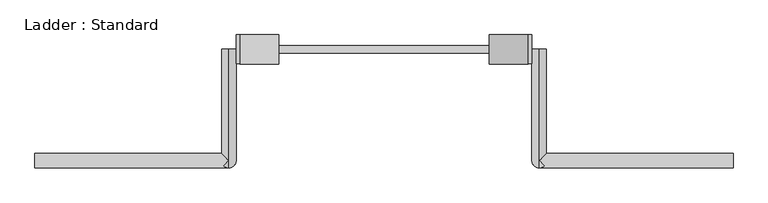
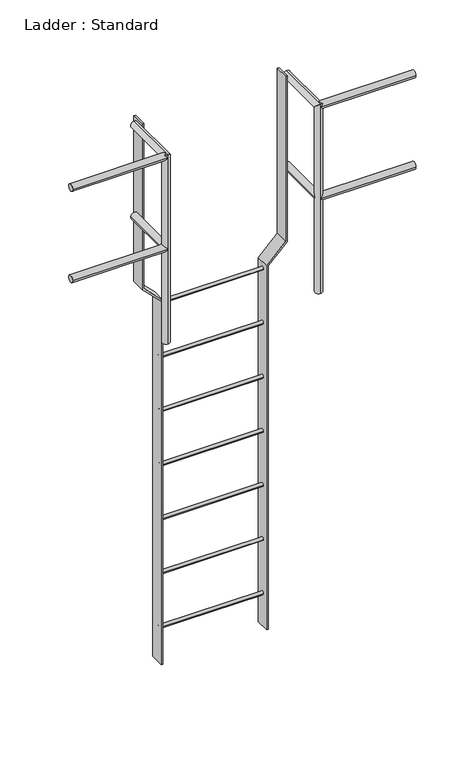
"""IFC4 building model written with IfcOpenShell, lengths in millimetres: proxy geometry, Ladder : Standard."""

import ifcopenshell
import ifcopenshell.guid

model = None  # the IFC model being written
_history = None  # IfcOwnerHistory: only IFC2X3 demands one
_inside = {}  # id of a spatial element -> (the spatial element, [elements in it])
_under = {}  # id of a project, library or spatial element -> (it, [spatial elements below it])
_declared = {}  # id of a project -> (the project, [libraries it declares])
_typed = {}  # id of a type object -> (the type object, [elements of that type])
_made_of = {}  # id of a material, layer set ... -> (it, [elements and type objects made of it])


def new_model(schema):
    """Start an empty IFC model of exactly this schema.

    Asked for "IFC4X3", IfcOpenShell would pick the latest addendum, in which some entities
    have other attributes; the version numbers below select the first issue.
    IFC2X3 requires an IfcOwnerHistory on every rooted entity: one is made here for all.
    """
    global model, _history
    if schema == "IFC4X3":
        model = ifcopenshell.file(schema_version=(4, 3, 0, 0))
    else:
        model = ifcopenshell.file(schema=schema)
    _inside.clear()
    _under.clear()
    _declared.clear()
    _typed.clear()
    _made_of.clear()
    _history = None
    if model.schema == "IFC2X3":
        org = make("IfcOrganization", Name="unknown")
        user = make(
            "IfcPersonAndOrganization",
            ThePerson=make("IfcPerson", FamilyName="unknown"),
            TheOrganization=org,
        )
        app = make(
            "IfcApplication",
            ApplicationDeveloper=org,
            Version="unknown",
            ApplicationFullName="unknown",
            ApplicationIdentifier="unknown",
        )
        _history = make(
            "IfcOwnerHistory",
            OwningUser=user,
            OwningApplication=app,
            ChangeAction="ADDED",
            CreationDate=0,
        )
    return model


def make(cls, **values):
    """One entity of the class cls with the attributes given. An attribute that is None is left unset."""
    return model.create_entity(
        cls, **{name: value for name, value in values.items() if value is not None}
    )


def rooted(cls, **values):
    """An entity with a GlobalId (a new one), such as an element, a storey or a relation."""
    return make(cls, GlobalId=ifcopenshell.guid.new(), OwnerHistory=_history, **values)


def si_unit(unit_type, name, prefix=None):
    """IfcSIUnit, for example si_unit("LENGTHUNIT", "METRE", prefix="MILLI")."""
    return make("IfcSIUnit", UnitType=unit_type, Prefix=prefix, Name=name)


def assignment(units):
    """IfcUnitAssignment: the units of a project."""
    return None if units is None else make("IfcUnitAssignment", Units=units)


def point(xyz):
    """IfcCartesianPoint."""
    return None if xyz is None else make("IfcCartesianPoint", Coordinates=xyz)


def direction(xyz):
    """IfcDirection."""
    return None if xyz is None else make("IfcDirection", DirectionRatios=xyz)


def frame(location, z_axis=None, x_axis=None):
    """IfcAxis2Placement3D, a coordinate frame: its origin and axes. An axis left out is left unset."""
    return make(
        "IfcAxis2Placement3D",
        Location=point(location),
        Axis=direction(z_axis),
        RefDirection=direction(x_axis),
    )


def frame_2d(location, x_axis=None):
    """IfcAxis2Placement2D, a coordinate frame in the plane: its origin and x axis."""
    return make(
        "IfcAxis2Placement2D", Location=point(location), RefDirection=direction(x_axis)
    )


def origin():
    """The frame at (0, 0, 0) with its axes left unset."""
    return frame((0.0, 0.0, 0.0))


def place(relative_to, where):
    """IfcLocalPlacement: puts the frame where relative to a parent placement (None: the world)."""
    return make(
        "IfcLocalPlacement", PlacementRelTo=relative_to, RelativePlacement=where
    )


def context(
    kind, dimensions, precision=None, world=None, true_north=None, identifier=None
):
    """IfcGeometricRepresentationContext, for example the 3D "Model" context."""
    return make(
        "IfcGeometricRepresentationContext",
        ContextIdentifier=identifier,
        ContextType=kind,
        CoordinateSpaceDimension=dimensions,
        Precision=precision,
        WorldCoordinateSystem=world,
        TrueNorth=true_north,
    )


def project(units=None, contexts=None):
    """IfcProject with its units and contexts."""
    return rooted(
        "IfcProject",
        Name="project",
        RepresentationContexts=contexts,
        UnitsInContext=assignment(units),
    )


def spatial(cls, under=None, at=None, **own):
    """A site, building, storey or space (cls), placed at a placement, below another one or the project."""
    s = rooted(cls, ObjectPlacement=at, **own)
    if under is not None:
        _under.setdefault(under.id(), (under, []))[1].append(s)
    return s


def polyline(points):
    """IfcPolyline through the points."""
    return make("IfcPolyline", Points=[point(p) for p in points])


def circle_curve(where, radius):
    """IfcCircle in the frame where."""
    return make("IfcCircle", Position=where, Radius=radius)


def ellipse_curve(where, semi_axis1, semi_axis2):
    """IfcEllipse in the frame where."""
    return make(
        "IfcEllipse", Position=where, SemiAxis1=semi_axis1, SemiAxis2=semi_axis2
    )


def trimmed(basis, trim1, trim2, sense, master):
    """IfcTrimmedCurve: the piece of a basis curve between two trims."""
    return make(
        "IfcTrimmedCurve",
        BasisCurve=basis,
        Trim1=trim1,
        Trim2=trim2,
        SenseAgreement=sense,
        MasterRepresentation=master,
    )


def segment(curve, same_sense, transition):
    """IfcCompositeCurveSegment."""
    return make(
        "IfcCompositeCurveSegment",
        Transition=transition,
        SameSense=same_sense,
        ParentCurve=curve,
    )


def composite_curve(segments, self_intersect=None):
    """IfcCompositeCurve: segments joined end to end."""
    return make("IfcCompositeCurve", Segments=segments, SelfIntersect=self_intersect)


def outline(outer, holes=None, kind="AREA"):
    """IfcArbitraryClosedProfileDef: a profile drawn as a closed curve; with holes, ...WithVoids."""
    if holes is None:
        return make("IfcArbitraryClosedProfileDef", ProfileType=kind, OuterCurve=outer)
    return make(
        "IfcArbitraryProfileDefWithVoids",
        ProfileType=kind,
        OuterCurve=outer,
        InnerCurves=holes,
    )


def extrude(swept, where, along, depth):
    """IfcExtrudedAreaSolid: the profile swept, set in the frame where, extruded along a direction by depth."""
    return make(
        "IfcExtrudedAreaSolid",
        SweptArea=swept,
        Position=where,
        ExtrudedDirection=direction(along),
        Depth=depth,
    )


def shape(context_of_items, identifier, shape_type, items):
    """IfcShapeRepresentation: the items that make up one representation, for example the "Body"."""
    return make(
        "IfcShapeRepresentation",
        ContextOfItems=context_of_items,
        RepresentationIdentifier=identifier,
        RepresentationType=shape_type,
        Items=items,
    )


def source(mapping_origin, context_of_items, identifier, shape_type, items):
    """IfcRepresentationMap: a shape defined once, which mapped items show again and again."""
    return make(
        "IfcRepresentationMap",
        MappingOrigin=mapping_origin,
        MappedRepresentation=shape(context_of_items, identifier, shape_type, items),
    )


def transform(
    local_origin,
    x_axis=None,
    y_axis=None,
    z_axis=None,
    scale=None,
    scale2=None,
    scale3=None,
    uniform=True,
):
    """IfcCartesianTransformationOperator3D, or its non-uniform kind. x_axis, y_axis, z_axis: its Axis1, 2, 3."""
    if uniform:
        return make(
            "IfcCartesianTransformationOperator3D",
            Axis1=direction(x_axis),
            Axis2=direction(y_axis),
            LocalOrigin=point(local_origin),
            Scale=scale,
            Axis3=direction(z_axis),
        )
    return make(
        "IfcCartesianTransformationOperator3DnonUniform",
        Axis1=direction(x_axis),
        Axis2=direction(y_axis),
        LocalOrigin=point(local_origin),
        Scale=scale,
        Axis3=direction(z_axis),
        Scale2=scale2,
        Scale3=scale3,
    )


def mapped(mapping_source, mapping_target):
    """IfcMappedItem: shows the shape of a source again, moved by a transform."""
    return make(
        "IfcMappedItem", MappingSource=mapping_source, MappingTarget=mapping_target
    )


def made_of(thing, what):
    """Note that an element or type object is made of a material, layer set ...; save() writes the relation."""
    if what is not None:
        _made_of.setdefault(what.id(), (what, []))[1].append(thing)
    return thing


def element(
    cls,
    number,
    at=None,
    inside=None,
    cuts=None,
    type_object=None,
    material=None,
    context=None,
    identifier="Body",
    shape_type=None,
    held_by="IfcProductDefinitionShape",
    body=None,
    shapes=None,
    **own,
):
    """One element of the class cls, such as IfcWall. Its Tag is "e" and its number.

    at: its placement. inside: the storey or other place that contains it. cuts: it is an
    opening in that element (IfcRelVoidsElement). A single representation is given by context,
    identifier, shape_type and body (its items); several are given by shapes. held_by: the class
    of the entity that holds the representations. save() writes the other relations.
    """
    e = rooted(cls, Tag="e%d" % number, ObjectPlacement=at, **own)
    if body is not None:
        shapes = [shape(context, identifier, shape_type, body)]
    if shapes is not None:
        e.Representation = make(held_by, Representations=shapes)
    if inside is not None:
        _inside.setdefault(inside.id(), (inside, []))[1].append(e)
    if cuts is not None:
        rooted(
            "IfcRelVoidsElement", RelatingBuildingElement=cuts, RelatedOpeningElement=e
        )
    if type_object is not None:
        _typed.setdefault(type_object.id(), (type_object, []))[1].append(e)
    return made_of(e, material)


def aggregate(whole, parts):
    """IfcRelAggregates: a whole, such as a stair, and the parts it consists of."""
    return rooted("IfcRelAggregates", RelatingObject=whole, RelatedObjects=parts)


def save(model, path):
    """Write the relations noted so far, then the file.

    IfcRelAggregates (storeys below a building ...), IfcRelContainedInSpatialStructure (elements
    in a storey), IfcRelDefinesByType, IfcRelAssociatesMaterial and IfcRelDeclares: one each for
    every whole, place, type object, material and project.
    """
    for whole, parts in _under.values():
        aggregate(whole, parts)
    for where, things in _inside.values():
        rooted(
            "IfcRelContainedInSpatialStructure",
            RelatedElements=things,
            RelatingStructure=where,
        )
    for kind, things in _typed.values():
        rooted("IfcRelDefinesByType", RelatedObjects=things, RelatingType=kind)
    for what, things in _made_of.values():
        rooted("IfcRelAssociatesMaterial", RelatedObjects=things, RelatingMaterial=what)
    for by, libraries in _declared.values():
        rooted("IfcRelDeclares", RelatingContext=by, RelatedDefinitions=libraries)
    model.write(path)


def plane_surface(at):
    """IfcPlane: the flat surface through the origin of the frame at, square to its z axis."""
    return make("IfcPlane", Position=at)


def cylinder_surface(at, radius):
    """IfcCylindricalSurface: all points at the distance radius from the z axis of the frame at."""
    return make("IfcCylindricalSurface", Position=at, Radius=radius)


def advanced_brep(points, edges, surfaces, faces):
    """IfcAdvancedBrep: a solid bounded by faces that lie on surfaces and meet in shared edges.

    An edge is (start, end): straight between two places in points (the first is 0);
    or (start, end, curve); or (start, end, curve, False) where it runs against its curve.
    A face is (place in surfaces, loops), or (place, loops, False) where it looks against
    its surface's normal. A loop lists edges by number (the first is 1), with a minus sign
    where the edge is run from its end to its start. The first loop is the outer one.
    """
    corners = [point(p) for p in points]
    vertices = [make("IfcVertexPoint", VertexGeometry=c) for c in corners]
    made = []
    for start, end, *more in edges:
        made.append(
            make(
                "IfcEdgeCurve",
                EdgeStart=vertices[start],
                EdgeEnd=vertices[end],
                EdgeGeometry=more[0] if more else make("IfcPolyline", Points=[corners[start], corners[end]]),
                SameSense=more[1] if len(more) > 1 else True,
            )
        )
    hull = []
    for where, loops, *sense in faces:
        bounds = []
        for j, loop in enumerate(loops):
            ring = [make("IfcOrientedEdge", EdgeElement=made[abs(k) - 1], Orientation=k > 0) for k in loop]
            bounds.append(
                make(
                    "IfcFaceOuterBound" if j == 0 else "IfcFaceBound",
                    Bound=make("IfcEdgeLoop", EdgeList=ring),
                    Orientation=True,
                )
            )
        hull.append(make("IfcAdvancedFace", Bounds=bounds, FaceSurface=surfaces[where], SameSense=sense[0] if sense else True))
    return make("IfcAdvancedBrep", Outer=make("IfcClosedShell", CfsFaces=hull))


def ladder_standard_c970834c(model_context):
    return source(origin(), model_context, "Body", "SolidModel", [
        extrude(outline(composite_curve([segment(trimmed(circle_curve(frame_2d((292.1, -1828.8)), 9.525), [point((282.575, -1828.8))], [point((301.625, -1828.8))], False, "CARTESIAN"), True, "CONTINUOUS"), segment(trimmed(circle_curve(frame_2d((292.1, -1828.8)), 9.525), [point((301.625, -1828.8))], [point((282.575, -1828.8))], False, "CARTESIAN"), True, "CONTINUOUS")], self_intersect=False)), frame((-276.3329351, 0.0, 0.0), z_axis=(1.0, 0.0, 0.0), x_axis=(0.0, 1.0, 0.0)), (0.0, 0.0, 1.0), 552.6658703),
        extrude(outline(composite_curve([segment(trimmed(circle_curve(frame_2d((292.1, -1524.0)), 9.525), [point((282.575, -1524.0))], [point((301.625, -1524.0))], False, "CARTESIAN"), True, "CONTINUOUS"), segment(trimmed(circle_curve(frame_2d((292.1, -1524.0)), 9.525), [point((301.625, -1524.0))], [point((282.575, -1524.0))], False, "CARTESIAN"), True, "CONTINUOUS")], self_intersect=False)), frame((-276.3329351, 0.0, 0.0), z_axis=(1.0, 0.0, 0.0), x_axis=(0.0, 1.0, 0.0)), (0.0, 0.0, 1.0), 552.6658703),
        extrude(outline(composite_curve([segment(trimmed(circle_curve(frame_2d((292.1, -1219.2)), 9.525), [point((282.575, -1219.2))], [point((301.625, -1219.2))], False, "CARTESIAN"), True, "CONTINUOUS"), segment(trimmed(circle_curve(frame_2d((292.1, -1219.2)), 9.525), [point((301.625, -1219.2))], [point((282.575, -1219.2))], False, "CARTESIAN"), True, "CONTINUOUS")], self_intersect=False)), frame((-276.3329351, 0.0, 0.0), z_axis=(1.0, 0.0, 0.0), x_axis=(0.0, 1.0, 0.0)), (0.0, 0.0, 1.0), 552.6658703),
        extrude(outline(composite_curve([segment(trimmed(circle_curve(frame_2d((292.1, -914.4)), 9.525), [point((282.575, -914.4))], [point((301.625, -914.4))], False, "CARTESIAN"), True, "CONTINUOUS"), segment(trimmed(circle_curve(frame_2d((292.1, -914.4)), 9.525), [point((301.625, -914.4))], [point((282.575, -914.4))], False, "CARTESIAN"), True, "CONTINUOUS")], self_intersect=False)), frame((-276.3329351, 0.0, 0.0), z_axis=(1.0, 0.0, 0.0), x_axis=(0.0, 1.0, 0.0)), (0.0, 0.0, 1.0), 552.6658703),
        extrude(outline(composite_curve([segment(trimmed(circle_curve(frame_2d((292.1, -609.6)), 9.525), [point((282.575, -609.6))], [point((301.625, -609.6))], False, "CARTESIAN"), True, "CONTINUOUS"), segment(trimmed(circle_curve(frame_2d((292.1, -609.6)), 9.525), [point((301.625, -609.6))], [point((282.575, -609.6))], False, "CARTESIAN"), True, "CONTINUOUS")], self_intersect=False)), frame((-276.3329351, 0.0, 0.0), z_axis=(1.0, 0.0, 0.0), x_axis=(0.0, 1.0, 0.0)), (0.0, 0.0, 1.0), 552.6658703),
        extrude(outline(composite_curve([segment(trimmed(circle_curve(frame_2d((292.1, -304.8)), 9.525), [point((282.575, -304.8))], [point((301.625, -304.8))], False, "CARTESIAN"), True, "CONTINUOUS"), segment(trimmed(circle_curve(frame_2d((292.1, -304.8)), 9.525), [point((301.625, -304.8))], [point((282.575, -304.8))], False, "CARTESIAN"), True, "CONTINUOUS")], self_intersect=False)), frame((-276.3329351, 0.0, 0.0), z_axis=(1.0, 0.0, 0.0), x_axis=(0.0, 1.0, 0.0)), (0.0, 0.0, 1.0), 552.6658703),
        extrude(outline(composite_curve([segment(trimmed(circle_curve(frame_2d((292.1, 0.0)), 9.525), [point((282.575, 0.0))], [point((301.625, 0.0))], False, "CARTESIAN"), True, "CONTINUOUS"), segment(trimmed(circle_curve(frame_2d((292.1, 0.0)), 9.525), [point((301.625, 0.0))], [point((282.575, 0.0))], False, "CARTESIAN"), True, "CONTINUOUS")], self_intersect=False)), frame((-276.3329351, 0.0, 0.0), z_axis=(1.0, 0.0, 0.0), x_axis=(0.0, 1.0, 0.0)), (0.0, 0.0, 1.0), 552.6658703),
        advanced_brep(
        [(387.4579351, 292.1, 533.4), (425.5579351, 292.1, 533.4), (425.5579351, 19.05, 533.4), (419.9783193, 13.4703842, 519.9296158), (406.5079351, 19.05, 514.35), (387.4579351, 0.0, 533.4), (406.5079351, 19.05, 552.45), (419.9783193, 13.4703842, 546.8703842), (914.5079351, -19.05, 533.4), (914.5079351, 19.05, 533.4), (406.5079351, -19.05, 533.4), (406.5079351, 19.05, 0.0), (406.5079351, -19.05, 0.0), (406.5079351, 19.05, 1028.7), (419.9783193, 13.4703842, 1034.2796158), (406.5079351, -19.05, 1047.75), (419.9783193, -13.4703842, 1061.2203842), (406.5079351, -19.05, 1066.8), (406.5079351, 292.1, 1028.7), (406.5079351, 292.1, 1066.8), (406.5079351, 0.0, 1066.8), (425.5579351, 19.05, 1047.75), (914.5079351, -19.05, 1047.75), (914.5079351, 19.05, 1047.75)],
        [
            (0, 1, circle_curve(frame((406.5079351, 292.1, 533.4), z_axis=(0.0, 1.0, 0.0), x_axis=(1.0, 0.0, 0.0)), 19.05)),
            (1, 0, circle_curve(frame((406.5079351, 292.1, 533.4), z_axis=(0.0, 1.0, 0.0), x_axis=(1.0, 0.0, 0.0)), 19.05)),
            (1, 2),
            (2, 3, ellipse_curve(frame((406.5079351, 0.0, 533.4), z_axis=(-0.7071067811865459, 0.7071067811865492, 0.0), x_axis=(-0.7071067811865492, -0.7071067811865457, 0.0)), 26.9407684, 19.05)),
            (3, 4, ellipse_curve(frame((406.5079351, 0.0, 533.4), z_axis=(0.0, 0.7071067811865475, 0.7071067811865475), x_axis=(0.0, -0.7071067811865476, 0.7071067811865474)), 26.9407684, 19.05)),
            (4, 5, ellipse_curve(frame((406.5079351, 0.0, 533.4), z_axis=(0.0, 0.7071067811865475, 0.7071067811865475), x_axis=(0.0, -0.7071067811865476, 0.7071067811865474)), 26.9407684, 19.05)),
            (5, 0),
            (5, 6, ellipse_curve(frame((406.5079351, 0.0, 533.4), z_axis=(0.0, 0.7071067811865475, -0.7071067811865475), x_axis=(0.0, -0.7071067811865476, -0.7071067811865474)), 26.9407684, 19.05)),
            (6, 7, ellipse_curve(frame((406.5079351, 0.0, 533.4), z_axis=(0.0, 0.7071067811865475, -0.7071067811865475), x_axis=(0.0, -0.7071067811865476, -0.7071067811865474)), 26.9407684, 19.05)),
            (7, 2, ellipse_curve(frame((406.5079351, 0.0, 533.4), z_axis=(-0.7071067811865459, 0.7071067811865492, 0.0), x_axis=(-0.7071067811865492, -0.7071067811865457, 0.0)), 26.9407684, 19.05)),
            (8, 9, circle_curve(frame((914.5079351, 0.0, 533.4), z_axis=(1.0, 0.0, 0.0), x_axis=(0.0, 1.0, 0.0)), 19.05)),
            (9, 8, circle_curve(frame((914.5079351, 0.0, 533.4), z_axis=(1.0, 0.0, 0.0), x_axis=(0.0, 1.0, 0.0)), 19.05)),
            (8, 10),
            (10, 3, ellipse_curve(frame((406.5079351, 0.0, 533.4), z_axis=(0.7071067811865475, 0.0, 0.7071067811865476), x_axis=(0.7071067811865476, 0.0, -0.7071067811865474)), 26.9407684, 19.05)),
            (2, 9),
            (7, 10, ellipse_curve(frame((406.5079351, 0.0, 533.4), z_axis=(0.7071067811865476, 0.0, -0.7071067811865475), x_axis=(0.7071067811865474, 0.0, 0.7071067811865476)), 26.9407684, 19.05)),
            (11, 12, circle_curve(frame((406.5079351, 0.0, 0.0), z_axis=(0.0, 0.0, -1.0), x_axis=(0.0, -1.0, 0.0)), 19.05)),
            (12, 11, circle_curve(frame((406.5079351, 0.0, 0.0), z_axis=(0.0, 0.0, -1.0), x_axis=(0.0, -1.0, 0.0)), 19.05)),
            (11, 4),
            (10, 12),
            (6, 13),
            (13, 14, ellipse_curve(frame((406.5079351, 0.0, 1047.75), z_axis=(0.0, -0.7071067811865475, -0.7071067811865475), x_axis=(0.0, 0.7071067811865474, -0.7071067811865476)), 26.9407684, 19.05)),
            (14, 15, ellipse_curve(frame((406.5079351, 0.0, 1047.75), z_axis=(-0.7071067811865475, 0.0, -0.7071067811865476), x_axis=(0.7071067811865476, 0.0, -0.7071067811865474)), 26.9407684, 19.05)),
            (15, 10),
            (16, 17, ellipse_curve(frame((406.5079351, 0.0, 1047.75), z_axis=(0.0, -0.7071067811865475, -0.7071067811865475), x_axis=(0.0, 0.7071067811865474, -0.7071067811865476)), 26.9407684, 19.05)),
            (17, 15),
            (15, 16, ellipse_curve(frame((406.5079351, 0.0, 1047.75), z_axis=(-0.7071067811865476, 0.0, 0.7071067811865475), x_axis=(-0.7071067811865474, 0.0, -0.7071067811865476)), 26.9407684, 19.05)),
            (17, 13, ellipse_curve(frame((406.5079351, 0.0, 1047.75), z_axis=(0.0, -0.7071067811865475, -0.7071067811865475), x_axis=(0.0, 0.7071067811865474, -0.7071067811865476)), 26.9407684, 19.05)),
            (18, 19, circle_curve(frame((406.5079351, 292.1, 1047.75), z_axis=(0.0, 1.0, 0.0), x_axis=(0.0, 0.0, 1.0)), 19.05)),
            (19, 18, circle_curve(frame((406.5079351, 292.1, 1047.75), z_axis=(0.0, 1.0, 0.0), x_axis=(0.0, 0.0, 1.0)), 19.05)),
            (16, 20, ellipse_curve(frame((406.5079351, 0.0, 1047.75), z_axis=(-0.7071067811865508, -0.7071067811865441, 0.0), x_axis=(0.7071067811865441, -0.7071067811865509, 0.0)), 26.9407684, 19.05)),
            (20, 17),
            (19, 20),
            (20, 21, ellipse_curve(frame((406.5079351, 0.0, 1047.75), z_axis=(-0.7071067811865441, 0.7071067811865508, 0.0), x_axis=(-0.7071067811865507, -0.7071067811865442, 0.0)), 26.9407684, 19.05)),
            (21, 14, ellipse_curve(frame((406.5079351, 0.0, 1047.75), z_axis=(-0.7071067811865441, 0.7071067811865508, 0.0), x_axis=(-0.7071067811865507, -0.7071067811865442, 0.0)), 26.9407684, 19.05)),
            (13, 18),
            (22, 23, circle_curve(frame((914.5079351, 0.0, 1047.75), z_axis=(1.0, 0.0, 0.0), x_axis=(0.0, 1.0, 0.0)), 19.05)),
            (23, 22, circle_curve(frame((914.5079351, 0.0, 1047.75), z_axis=(1.0, 0.0, 0.0), x_axis=(0.0, 1.0, 0.0)), 19.05)),
            (22, 15),
            (21, 23),
        ],
        [
            plane_surface(frame((425.5579351, 292.1, 533.4), z_axis=(0.0, 1.0, 0.0), x_axis=(0.0, 0.0, -1.0))),
            cylinder_surface(frame((406.5079351, 292.1, 533.4), z_axis=(0.0, -1.0, 0.0), x_axis=(1.0, 0.0, 0.0)), 19.05),
            plane_surface(frame((914.5079351, 19.05, 533.4), z_axis=(1.0, 0.0, 0.0), x_axis=(0.0, 0.0, 1.0))),
            cylinder_surface(frame((406.5079351, 0.0, 533.4), z_axis=(1.0, 0.0, 0.0), x_axis=(0.0, 1.0, 0.0)), 19.05),
            plane_surface(frame((0.0, 0.0, 0.0), z_axis=(0.0, 0.0, -1.0), x_axis=(1.0, 0.0, 0.0))),
            cylinder_surface(frame((406.5079351, 0.0, 0.0), z_axis=(0.0, 0.0, -1.0), x_axis=(0.0, -1.0, 0.0)), 19.05),
            plane_surface(frame((0.0, 292.1, 1047.75), z_axis=(0.0, 1.0, 0.0), x_axis=(1.0, 0.0, 0.0))),
            cylinder_surface(frame((406.5079351, 0.0, 1047.75), z_axis=(0.0, -1.0, 0.0), x_axis=(0.0, 0.0, 1.0)), 19.05),
            plane_surface(frame((914.5079351, 19.05, 1047.75), z_axis=(1.0, 0.0, 0.0), x_axis=(0.0, 0.0, 1.0))),
            cylinder_surface(frame((406.5079351, 0.0, 1047.75), z_axis=(1.0, 0.0, 0.0), x_axis=(0.0, 1.0, 0.0)), 19.05),
        ],
        [
            (0, [[1, 2]]),
            (1, [[-2, 3, 4, 5, 6, 7]]),
            (1, [[-1, -7, 8, 9, 10, -3]]),
            (2, [[11, 12]]),
            (3, [[-11, 13, 14, -4, 15]]),
            (3, [[-12, -15, -10, 16, -13]]),
            (4, [[17, 18]]),
            (5, [[-17, 19, -5, -14, 20]]),
            (5, [[21, 22, 23, 24, -16, -9]]),
            (5, [[25, 26, 27]]),
            (5, [[-18, -20, -24, -26, 28, -21, -8, -6, -19]]),
            (6, [[29, 30]]),
            (7, [[-25, 31, 32]]),
            (7, [[-30, 33, 34, 35, -22, 36]]),
            (7, [[-28, -32, -33, -29, -36]]),
            (8, [[37, 38]]),
            (9, [[-37, 39, -23, -35, 40]]),
            (9, [[-38, -40, -34, -31, -27, -39]]),
        ],
    ),
        advanced_brep(
        [(-914.5079351, -19.05, 533.4), (-914.5079351, 19.05, 533.4), (-425.5579351, 19.05, 533.4), (-419.9783193, 13.4703842, 519.9296158), (-406.5079351, -19.05, 533.4), (-419.9783193, 13.4703842, 546.8703842), (-425.5579351, 292.1, 533.4), (-387.4579351, 292.1, 533.4), (-387.4579351, 0.0, 533.4), (-406.5079351, 19.05, 514.35), (-406.5079351, 19.05, 552.45), (-406.5079351, 19.05, 0.0), (-406.5079351, -19.05, 0.0), (-406.5079351, 19.05, 1028.7), (-406.5079351, -19.05, 1066.8), (-406.5079351, -19.05, 1047.75), (-419.9783193, 13.4703842, 1034.2796158), (-419.9783193, -13.4703842, 1061.2203842), (-406.5079351, 292.1, 1028.7), (-406.5079351, 292.1, 1066.8), (-406.5079351, 0.0, 1066.8), (-425.5579351, 19.05, 1047.75), (-914.5079351, -19.05, 1047.75), (-914.5079351, 19.05, 1047.75)],
        [
            (0, 1, circle_curve(frame((-914.5079351, 0.0, 533.4), z_axis=(-1.0, 0.0, 0.0), x_axis=(0.0, 1.0, 0.0)), 19.05)),
            (1, 0, circle_curve(frame((-914.5079351, 0.0, 533.4), z_axis=(-1.0, 0.0, 0.0), x_axis=(0.0, 1.0, 0.0)), 19.05)),
            (1, 2),
            (2, 3, ellipse_curve(frame((-406.5079351, 0.0, 533.4), z_axis=(-0.7071067811865491, -0.7071067811865458, 0.0), x_axis=(0.7071067811865459, -0.707106781186549, 0.0)), 26.9407684, 19.05)),
            (3, 4, ellipse_curve(frame((-406.5079351, 0.0, 533.4), z_axis=(-0.7071067811865476, 0.0, 0.7071067811865475), x_axis=(0.7071067811865474, 0.0, 0.7071067811865476)), 26.9407684, 19.05)),
            (4, 0),
            (4, 5, ellipse_curve(frame((-406.5079351, 0.0, 533.4), z_axis=(-0.7071067811865475, 0.0, -0.7071067811865476), x_axis=(0.7071067811865476, 0.0, -0.7071067811865474)), 26.9407684, 19.05)),
            (5, 2, ellipse_curve(frame((-406.5079351, 0.0, 533.4), z_axis=(-0.7071067811865491, -0.7071067811865458, 0.0), x_axis=(0.7071067811865459, -0.707106781186549, 0.0)), 26.9407684, 19.05)),
            (6, 7, circle_curve(frame((-406.5079351, 292.1, 533.4), z_axis=(0.0, 1.0, 0.0), x_axis=(1.0, 0.0, 0.0)), 19.05)),
            (7, 6, circle_curve(frame((-406.5079351, 292.1, 533.4), z_axis=(0.0, 1.0, 0.0), x_axis=(1.0, 0.0, 0.0)), 19.05)),
            (7, 8),
            (8, 9, ellipse_curve(frame((-406.5079351, 0.0, 533.4), z_axis=(0.0, 0.7071067811865475, 0.7071067811865475), x_axis=(0.0, -0.7071067811865476, 0.7071067811865474)), 26.9407684, 19.05)),
            (9, 3, ellipse_curve(frame((-406.5079351, 0.0, 533.4), z_axis=(0.0, 0.7071067811865475, 0.7071067811865475), x_axis=(0.0, -0.7071067811865476, 0.7071067811865474)), 26.9407684, 19.05)),
            (2, 6),
            (5, 10, ellipse_curve(frame((-406.5079351, 0.0, 533.4), z_axis=(0.0, 0.7071067811865475, -0.7071067811865475), x_axis=(0.0, -0.7071067811865476, -0.7071067811865474)), 26.9407684, 19.05)),
            (10, 8, ellipse_curve(frame((-406.5079351, 0.0, 533.4), z_axis=(0.0, 0.7071067811865475, -0.7071067811865475), x_axis=(0.0, -0.7071067811865476, -0.7071067811865474)), 26.9407684, 19.05)),
            (11, 12, circle_curve(frame((-406.5079351, 0.0, 0.0), z_axis=(0.0, 0.0, -1.0), x_axis=(0.0, -1.0, 0.0)), 19.05)),
            (12, 11, circle_curve(frame((-406.5079351, 0.0, 0.0), z_axis=(0.0, 0.0, -1.0), x_axis=(0.0, -1.0, 0.0)), 19.05)),
            (11, 9),
            (10, 13),
            (13, 14, ellipse_curve(frame((-406.5079351, 0.0, 1047.75), z_axis=(0.0, -0.7071067811865475, -0.7071067811865475), x_axis=(0.0, 0.7071067811865474, -0.7071067811865476)), 26.9407684, 19.05)),
            (14, 15),
            (15, 4),
            (4, 12),
            (15, 16, ellipse_curve(frame((-406.5079351, 0.0, 1047.75), z_axis=(0.7071067811865476, 0.0, -0.7071067811865475), x_axis=(-0.7071067811865474, 0.0, -0.7071067811865476)), 26.9407684, 19.05)),
            (16, 13, ellipse_curve(frame((-406.5079351, 0.0, 1047.75), z_axis=(0.0, -0.7071067811865475, -0.7071067811865475), x_axis=(0.0, 0.7071067811865474, -0.7071067811865476)), 26.9407684, 19.05)),
            (14, 17, ellipse_curve(frame((-406.5079351, 0.0, 1047.75), z_axis=(0.0, -0.7071067811865475, -0.7071067811865475), x_axis=(0.0, 0.7071067811865474, -0.7071067811865476)), 26.9407684, 19.05)),
            (17, 15, ellipse_curve(frame((-406.5079351, 0.0, 1047.75), z_axis=(0.7071067811865475, 0.0, 0.7071067811865476), x_axis=(0.7071067811865476, 0.0, -0.7071067811865474)), 26.9407684, 19.05)),
            (18, 19, circle_curve(frame((-406.5079351, 292.1, 1047.75), z_axis=(0.0, 1.0, 0.0), x_axis=(0.0, 0.0, 1.0)), 19.05)),
            (19, 18, circle_curve(frame((-406.5079351, 292.1, 1047.75), z_axis=(0.0, 1.0, 0.0), x_axis=(0.0, 0.0, 1.0)), 19.05)),
            (13, 18),
            (19, 20),
            (20, 14),
            (20, 17, ellipse_curve(frame((-406.5079351, 0.0, 1047.75), z_axis=(0.7071067811865441, -0.7071067811865508, 0.0), x_axis=(-0.7071067811865507, -0.7071067811865442, 0.0)), 26.9407684, 19.05)),
            (16, 21, ellipse_curve(frame((-406.5079351, 0.0, 1047.75), z_axis=(0.7071067811865508, 0.7071067811865441, 0.0), x_axis=(0.7071067811865441, -0.7071067811865509, 0.0)), 26.9407684, 19.05)),
            (21, 20, ellipse_curve(frame((-406.5079351, 0.0, 1047.75), z_axis=(0.7071067811865508, 0.7071067811865441, 0.0), x_axis=(0.7071067811865441, -0.7071067811865509, 0.0)), 26.9407684, 19.05)),
            (22, 23, circle_curve(frame((-914.5079351, 0.0, 1047.75), z_axis=(-1.0, 0.0, 0.0), x_axis=(0.0, 1.0, 0.0)), 19.05)),
            (23, 22, circle_curve(frame((-914.5079351, 0.0, 1047.75), z_axis=(-1.0, 0.0, 0.0), x_axis=(0.0, 1.0, 0.0)), 19.05)),
            (23, 21),
            (15, 22),
        ],
        [
            plane_surface(frame((-914.5079351, 19.05, 533.4), z_axis=(-1.0, 0.0, 0.0), x_axis=(0.0, 0.0, -1.0))),
            cylinder_surface(frame((-914.5079351, 0.0, 533.4), z_axis=(1.0, 0.0, 0.0), x_axis=(0.0, 1.0, 0.0)), 19.05),
            plane_surface(frame((-387.4579351, 292.1, 533.4), z_axis=(0.0, 1.0, 0.0), x_axis=(0.0, 0.0, -1.0))),
            cylinder_surface(frame((-406.5079351, 292.1, 533.4), z_axis=(0.0, -1.0, 0.0), x_axis=(1.0, 0.0, 0.0)), 19.05),
            plane_surface(frame((0.0, 0.0, 0.0), z_axis=(0.0, 0.0, -1.0), x_axis=(1.0, 0.0, 0.0))),
            cylinder_surface(frame((-406.5079351, 0.0, 0.0), z_axis=(0.0, 0.0, -1.0), x_axis=(0.0, -1.0, 0.0)), 19.05),
            plane_surface(frame((0.0, 292.1, 1047.75), z_axis=(0.0, 1.0, 0.0), x_axis=(1.0, 0.0, 0.0))),
            cylinder_surface(frame((-406.5079351, 0.0, 1047.75), z_axis=(0.0, -1.0, 0.0), x_axis=(0.0, 0.0, 1.0)), 19.05),
            plane_surface(frame((-914.5079351, 19.05, 1047.75), z_axis=(-1.0, 0.0, 0.0), x_axis=(0.0, 0.0, -1.0))),
            cylinder_surface(frame((-914.5079351, 0.0, 1047.75), z_axis=(1.0, 0.0, 0.0), x_axis=(0.0, 1.0, 0.0)), 19.05),
        ],
        [
            (0, [[1, 2]]),
            (1, [[-2, 3, 4, 5, 6]]),
            (1, [[-1, -6, 7, 8, -3]]),
            (2, [[9, 10]]),
            (3, [[-10, 11, 12, 13, -4, 14]]),
            (3, [[-9, -14, -8, 15, 16, -11]]),
            (4, [[17, 18]]),
            (5, [[-17, 19, -12, -16, 20, 21, 22, 23, 24]]),
            (5, [[-18, -24, -5, -13, -19]]),
            (5, [[-20, -15, -7, -23, 25, 26]]),
            (5, [[27, 28, -22]]),
            (6, [[29, 30]]),
            (7, [[-21, 31, -30, 32, 33]]),
            (7, [[-27, -33, 34]]),
            (7, [[-29, -31, -26, 35, 36, -32]]),
            (8, [[37, 38]]),
            (9, [[-38, 39, -35, -25, 40]]),
            (9, [[-37, -40, -28, -34, -36, -39]]),
        ],
    ),
        extrude(outline(polyline([(1066.8, -387.4579351), (133.35, -387.4579351), (31.75, -285.8579351), (-2014.7139047, -285.8579351), (-2014.7139047, -276.3329351), (35.6953842, -276.3329351), (137.2953842, -377.9329351), (1066.8, -377.9329351), (1066.8, -387.4579351)])), frame((0.0, 254.0, 0.0), z_axis=(0.0, 1.0, 0.0), x_axis=(0.0, 0.0, 1.0)), (0.0, 0.0, 1.0), 76.2),
        extrude(outline(polyline([(1066.8, 377.9329351), (137.2953842, 377.9329351), (35.6953842, 276.3329351), (-2014.7139047, 276.3329351), (-2014.7139047, 285.8579351), (31.75, 285.8579351), (133.35, 387.4579351), (1066.8, 387.4579351), (1066.8, 377.9329351)])), frame((0.0, 254.0, 0.0), z_axis=(0.0, 1.0, 0.0), x_axis=(0.0, 0.0, 1.0)), (0.0, 0.0, 1.0), 76.2),
    ])


if __name__ == "__main__":
    model = new_model("IFC4")
    model_context = context("Model", 3, world=origin())
    ifc_project = project(units=[si_unit("LENGTHUNIT", "METRE", prefix="MILLI")], contexts=[model_context])
    site = spatial("IfcSite", under=ifc_project)
    building = spatial("IfcBuilding", under=site)
    placement = place(None, origin())
    ladder_standard_shape = ladder_standard_c970834c(model_context)
    element("IfcBuildingElementProxy", 1, Name="Ladder : Standard", ObjectType="Ladder : Standard", at=placement, inside=building, context=model_context, shape_type="MappedRepresentation", body=[
        mapped(ladder_standard_shape, transform((0.0, 0.0, 0.0), x_axis=(1.0, 0.0, 0.0), y_axis=(0.0, 1.0, 0.0), z_axis=(0.0, 0.0, 1.0))),
    ])
    save(model, "model.ifc")

# Revit data of these elements
# Type "Ladder : Standard"
#   Rung Radius = 9.525 mm
#   Rung Length [instance default] = 406.4 mm
#   Side Rail Thickness = 76.2 mm
#   Side Rail Width = 9.525 mm
#   Half Guardrail Height = 533.4 mm
#   Height [instance default] = 4635.5 mm
#   Guardrail Length = 508 mm
#   Guardrail Height = 1066.8 mm
#   Distance [instance default] = 177.8 mm
#   Rung Space [instance default] = 304.8 mm
#   Number of Rungs [instance default] = 15
#   Default Elevation = 0
# Element 1 (IfcBuildingElementProxy, "Ladder : Standard")
#   Rung Length = 552.666 mm
#   Height = 2014.714 mm
#   Number of Rungs = 7
